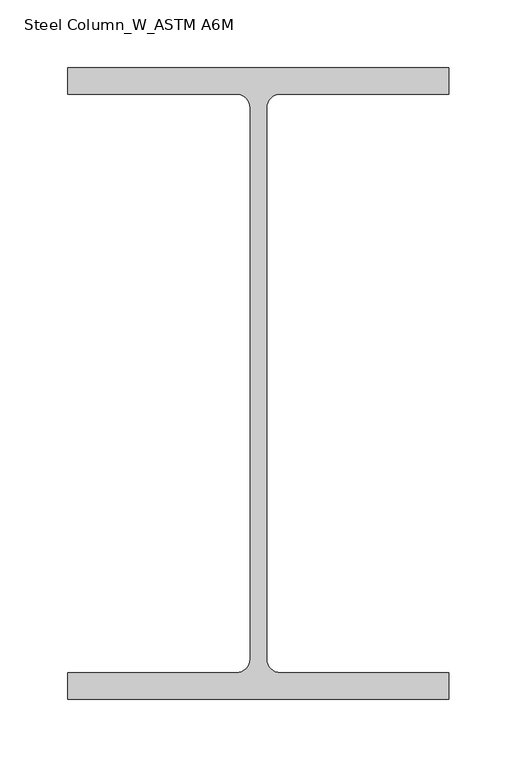
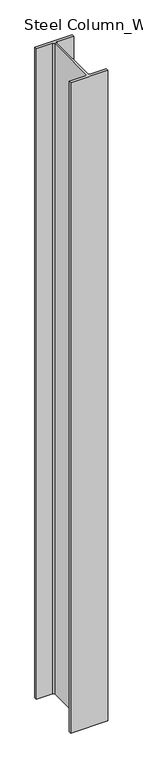
"""IFC4 building model written with IfcOpenShell, lengths in millimetres: column geometry, Steel Column_W_ASTM A6M : H_SC_AR_S01_W460x128_C1."""

from ifc_helpers import new_model, si_unit, point, frame, frame_2d, origin, place, context, project, spatial, polyline, circle_curve, trimmed, segment, composite_curve, outline, extrude, source, transform, mapped, element, save


def steel_column_w_astm_a6m_cc582183(model_context):
    return source(origin(), model_context, "Body", "SweptSolid", [
        extrude(outline(composite_curve([segment(polyline([(141.0, 233.5), (141.0, 213.9), (16.2, 213.9)]), True, "CONTINUOUS"), segment(trimmed(circle_curve(frame_2d((16.2, 203.8)), 10.1), [point((16.2, 213.9))], [point((6.1, 203.8))], True, "CARTESIAN"), True, "CONTINUOUS"), segment(polyline([(6.1, 203.8), (6.1, -203.8)]), True, "CONTINUOUS"), segment(trimmed(circle_curve(frame_2d((16.2, -203.8)), 10.1), [point((6.1, -203.8))], [point((16.2, -213.9))], True, "CARTESIAN"), True, "CONTINUOUS"), segment(polyline([(16.2, -213.9), (141.0, -213.9), (141.0, -233.5), (-141.0, -233.5), (-141.0, -213.9), (-16.2, -213.9)]), True, "CONTINUOUS"), segment(trimmed(circle_curve(frame_2d((-16.2, -203.8)), 10.1), [point((-16.2, -213.9))], [point((-6.1, -203.8))], True, "CARTESIAN"), True, "CONTINUOUS"), segment(polyline([(-6.1, -203.8), (-6.1, 203.8)]), True, "CONTINUOUS"), segment(trimmed(circle_curve(frame_2d((-16.2, 203.8)), 10.1), [point((-6.1, 203.8))], [point((-16.2, 213.9))], True, "CARTESIAN"), True, "CONTINUOUS"), segment(polyline([(-16.2, 213.9), (-141.0, 213.9), (-141.0, 233.5), (141.0, 233.5)]), True, "CONTINUOUS")], self_intersect=False)), frame((0.0, 0.0, 3519.8243501), z_axis=(0.0, 0.0, 1.0), x_axis=(1.0, 0.0, 0.0)), (0.0, 0.0, 1.0), 5200.0),
    ])


if __name__ == "__main__":
    model = new_model("IFC4")
    model_context = context("Model", 3, world=origin())
    ifc_project = project(units=[si_unit("LENGTHUNIT", "METRE", prefix="MILLI")], contexts=[model_context])
    site = spatial("IfcSite", under=ifc_project)
    building = spatial("IfcBuilding", under=site)
    placement = place(None, origin())
    steel_column_w_astm_a6m_shape = steel_column_w_astm_a6m_cc582183(model_context)
    element("IfcColumn", 1, ObjectType="Steel Column_W_ASTM A6M : H_SC_AR_S01_W460x128_C1", at=placement, inside=building, context=model_context, shape_type="MappedRepresentation", body=[
        mapped(steel_column_w_astm_a6m_shape, transform((0.0, 0.0, 0.0), x_axis=(1.0, 0.0, 0.0), y_axis=(0.0, 1.0, 0.0), z_axis=(0.0, 0.0, 1.0))),
    ])
    save(model, "model.ifc")

# Revit data of these elements
# Type "Steel Column_W_ASTM A6M : H_SC_AR_S01_W460x128_C1"
#   Section Name Key = "W18x86"
#   Width = 28.2 cm
#   Web Thickness = 1.22 cm
#   Web Fillet = 1.01 cm
#   Warping Constant = 3650000.0 cm⁶
#   Torsional Moment of Inertia = 171.00 cm⁴
#   Section Area = 163.0 cm²
#   Plastic Modulus weak axis = 793.0 cm³
#   Plastic Modulus strong axis = 3050.0 cm³
#   Perimeter = 2.02 m²/m
#   Nominal Weight = 128.00 kgf/m
#   Moment of Inertia weak axis = 7280.00 cm⁴
#   Moment of Inertia strong axis = 63700.00 cm⁴
#   Height = 46.7 cm
#   Flange Thickness = 1.96 cm
#   Elastic Modulus weak axis = 518.0 cm³
#   Elastic Modulus strong axis = 2720.0 cm³
#   Centroid Vertical = 23.35 cm
#   Centroid Horizontal = 14.1 cm
#   Structural Material [instance default] = Steel, 45-345
#   Bolt Spacing = 0
#   Assembly Code = ""
# Element 1 (IfcColumn, "Steel Column_W_ASTM A6M : H_SC_AR_S01_W460x128_C1")
#   Structural Material = Steel ASTM A992 GRADE 50
#   Materials on its faces: "Steel ASTM A992 GRADE 50"
# Materials
#   "Steel, 45-345": class "Metal", colour RGB 189 187 185, transparency 0, Description = "Steel 345 MPa", Cost = 0
#   "Steel ASTM A992 GRADE 50": class "Metal", colour RGB 120 120 120, transparency 0, Description = "Structural steel 50ksi", Cost = 0
